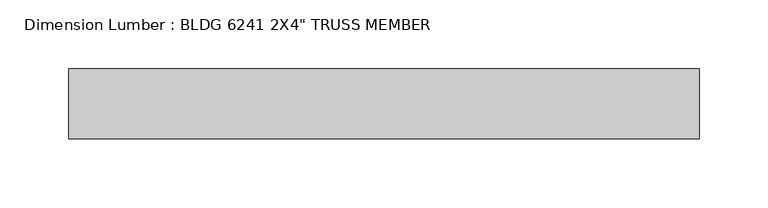
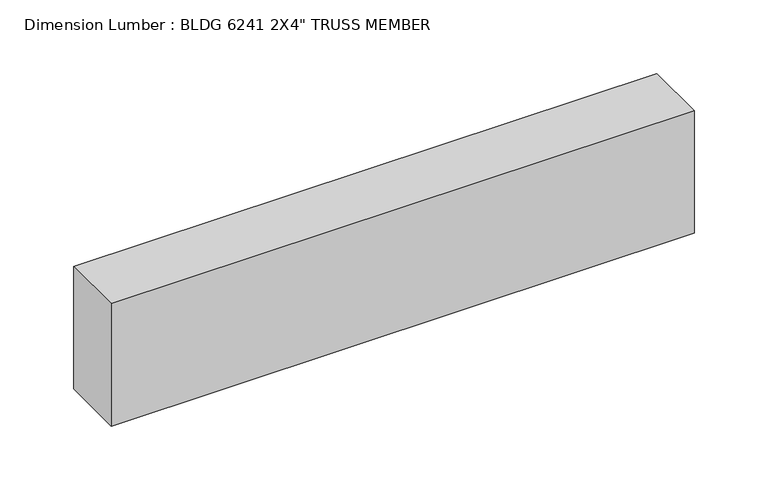
"""IFC4 building model written with IfcOpenShell, lengths in millimetres: beam geometry."""

from ifc_helpers import new_model, si_unit, frame, origin, place, context, project, spatial, polyline, outline, extrude, source, transform, mapped, element, save


def beam_b78a0881(model_context):
    return source(origin(), model_context, "Body", "SweptSolid", [
        extrude(outline(polyline([(228.6, 25.4), (228.6, -25.4), (-228.6, -25.4), (-228.6, 25.4), (228.6, 25.4)])), frame((0.0, 0.0, -50.8), z_axis=(0.0, 0.0, 1.0), x_axis=(1.0, 0.0, 0.0)), (0.0, 0.0, 1.0), 101.6),
    ])


if __name__ == "__main__":
    model = new_model("IFC4")
    model_context = context("Model", 3, world=origin())
    ifc_project = project(units=[si_unit("LENGTHUNIT", "METRE", prefix="MILLI")], contexts=[model_context])
    site = spatial("IfcSite", under=ifc_project)
    building = spatial("IfcBuilding", under=site)
    placement = place(None, origin())
    beam_shape = beam_b78a0881(model_context)
    element("IfcBeam", 1, ObjectType="Dimension Lumber : BLDG 6241 2X4\" TRUSS MEMBER", at=placement, inside=building, context=model_context, shape_type="MappedRepresentation", body=[
        mapped(beam_shape, transform((0.0, 0.0, 0.0), x_axis=(1.0, 0.0, 0.0), y_axis=(0.0, 1.0, 0.0), z_axis=(0.0, 0.0, 1.0))),
    ])
    save(model, "model.ifc")

# Revit data of these elements
# Type "Dimension Lumber : BLDG 6241 2X4\" TRUSS MEMBER"
#   Assembly Code = "B10"
#   A = 0.273472 SF
#   Length [instance default] = 5' - 0"
#   b = 0' - 2"
#   d = 0' - 4"
#   Structural Material [instance default] = Softwood, Lumber
# Element 1 (IfcBeam, "Dimension Lumber : BLDG 6241 2X4\" TRUSS MEMBER")
#   Materials on its faces: "Softwood, Lumber"
# Materials
#   "Softwood, Lumber": class "Wood", colour RGB 223 192 134, transparency 0, Description = "Pinus Echinata", Cost = 0
